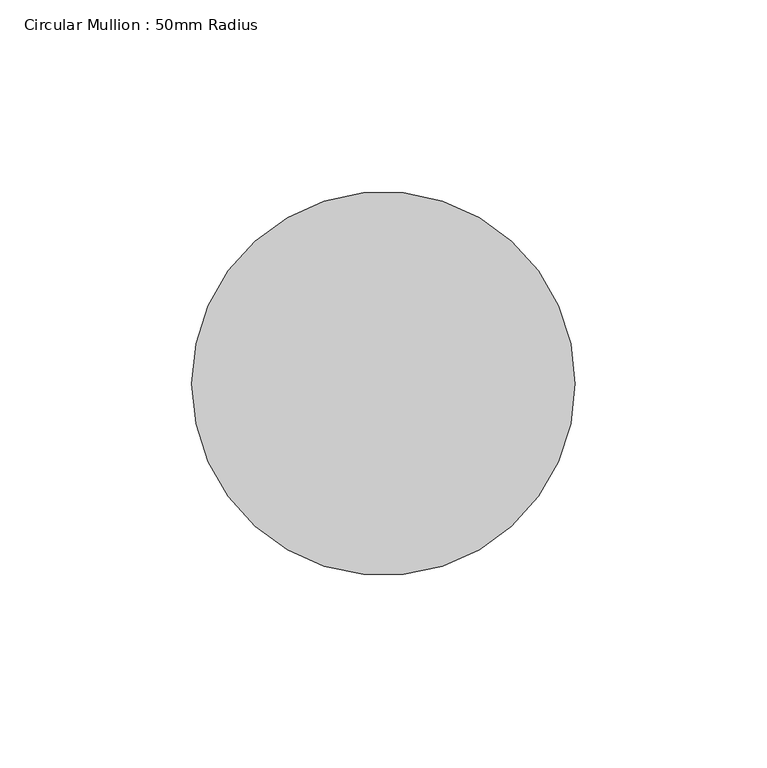
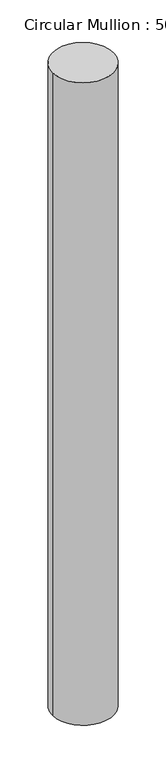
"""IFC4 building model written with IfcOpenShell, lengths in millimetres: member geometry, Circular Mullion : 50mm Radius."""

from ifc_helpers import new_model, si_unit, point, frame, origin, origin_2d, place, context, project, spatial, circle_curve, trimmed, segment, composite_curve, outline, extrude, source, transform, mapped, element, save


def circular_mullion_50mm_radius_bf215f65(model_context):
    return source(origin(), model_context, "Body", "SweptSolid", [
        extrude(outline(composite_curve([segment(trimmed(circle_curve(origin_2d(), 50.0), [point((50.0, 0.0))], [point((-50.0, 0.0))], False, "CARTESIAN"), True, "CONTINUOUS"), segment(trimmed(circle_curve(origin_2d(), 50.0), [point((-50.0, 0.0))], [point((50.0, 0.0))], False, "CARTESIAN"), True, "CONTINUOUS")], self_intersect=False)), frame((0.0, 0.0, -1116.1944087), z_axis=(0.0, 0.0, 1.0), x_axis=(1.0, 0.0, 0.0)), (0.0, 0.0, 1.0), 1116.1944087),
    ])


if __name__ == "__main__":
    model = new_model("IFC4")
    model_context = context("Model", 3, world=origin())
    ifc_project = project(units=[si_unit("LENGTHUNIT", "METRE", prefix="MILLI")], contexts=[model_context])
    site = spatial("IfcSite", under=ifc_project)
    building = spatial("IfcBuilding", under=site)
    placement = place(None, origin())
    circular_mullion_50mm_radius_shape = circular_mullion_50mm_radius_bf215f65(model_context)
    element("IfcMember", 1, ObjectType="Circular Mullion : 50mm Radius", at=placement, inside=building, context=model_context, shape_type="MappedRepresentation", body=[
        mapped(circular_mullion_50mm_radius_shape, transform((0.0, 0.0, 0.0), x_axis=(1.0, 0.0, 0.0), y_axis=(0.0, 1.0, 0.0), z_axis=(0.0, 0.0, 1.0))),
    ])
    save(model, "model.ifc")

# Revit data of these elements
# Type "Circular Mullion : 50mm Radius"
#   built-in parameter 1007350 = 0.164042 (stored number, unit not read)
# Element 1 (IfcMember, "Circular Mullion : 50mm Radius")
#   Materials on its faces: "Aluminium"
# Materials
#   "Aluminium": class "Metal", colour RGB 247 247 247, transparency 0, Description = "Aluminium 6061", Cost = 0
